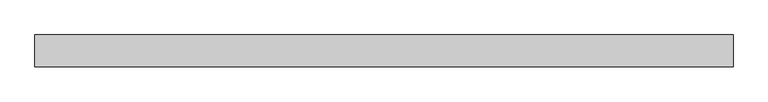
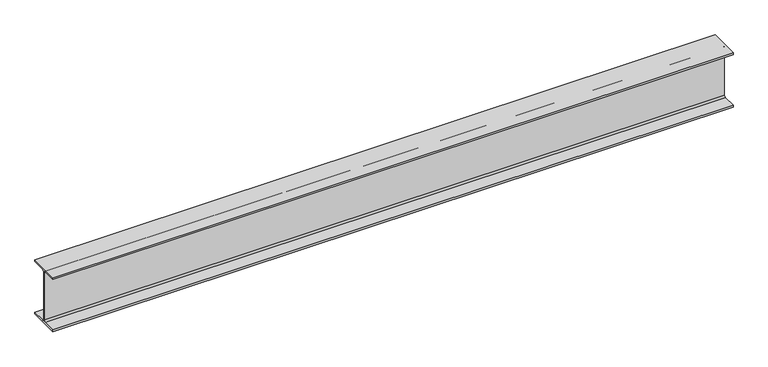
"""IFC4 building model written with IfcOpenShell, lengths in millimetres: beam geometry, Old_Steel Beam_H-KSD3502 : H_SB_ASB_H-200×200x8x12."""

from ifc_helpers import new_model, si_unit, point, frame, frame_2d, origin, place, context, project, spatial, polyline, circle_curve, trimmed, segment, composite_curve, outline, extrude, source, transform, mapped, element, save


def beam_a9061e91(model_context):
    return source(origin(), model_context, "Body", "SweptSolid", [
        extrude(outline(composite_curve([segment(polyline([(82.5, -141.5), (82.5, -151.7), (-82.5, -151.7), (-82.5, -141.5), (-11.9, -141.5)]), True, "CONTINUOUS"), segment(trimmed(circle_curve(frame_2d((-11.9, -132.6)), 8.9), [point((-11.9, -141.5))], [point((-3.0, -132.6))], True, "CARTESIAN"), True, "CONTINUOUS"), segment(polyline([(-3.0, -132.6), (-3.0, 132.6)]), True, "CONTINUOUS"), segment(trimmed(circle_curve(frame_2d((-11.9, 132.6)), 8.9), [point((-3.0, 132.6))], [point((-11.9, 141.5))], True, "CARTESIAN"), True, "CONTINUOUS"), segment(polyline([(-11.9, 141.5), (-82.5, 141.5), (-82.5, 151.7), (82.5, 151.7), (82.5, 141.5), (11.9, 141.5)]), True, "CONTINUOUS"), segment(trimmed(circle_curve(frame_2d((11.9, 132.6)), 8.9), [point((11.9, 141.5))], [point((3.0, 132.6))], True, "CARTESIAN"), True, "CONTINUOUS"), segment(polyline([(3.0, 132.6), (3.0, -132.6)]), True, "CONTINUOUS"), segment(trimmed(circle_curve(frame_2d((11.9, -132.6)), 8.9), [point((3.0, -132.6))], [point((11.9, -141.5))], True, "CARTESIAN"), True, "CONTINUOUS"), segment(polyline([(11.9, -141.5), (82.5, -141.5)]), True, "CONTINUOUS")], self_intersect=False)), frame((-1890.900922, 0.0, 0.0), z_axis=(1.0, 0.0, 0.0), x_axis=(0.0, 1.0, 0.0)), (0.0, 0.0, 1.0), 3596.321771),
    ])


if __name__ == "__main__":
    model = new_model("IFC4")
    model_context = context("Model", 3, world=origin())
    ifc_project = project(units=[si_unit("LENGTHUNIT", "METRE", prefix="MILLI")], contexts=[model_context])
    site = spatial("IfcSite", under=ifc_project)
    building = spatial("IfcBuilding", under=site)
    placement = place(None, origin())
    beam_shape = beam_a9061e91(model_context)
    element("IfcBeam", 1, ObjectType="Old_Steel Beam_H-KSD3502 : H_SB_ASB_H-200×200x8x12", at=placement, inside=building, context=model_context, shape_type="MappedRepresentation", body=[
        mapped(beam_shape, transform((0.0, 0.0, 0.0), x_axis=(1.0, 0.0, 0.0), y_axis=(0.0, 1.0, 0.0), z_axis=(0.0, 0.0, 1.0))),
    ])
    save(model, "model.ifc")

# Revit data of these elements
# Type "Old_Steel Beam_H-KSD3502 : H_SB_ASB_H-200×200x8x12"
#   Width = 20.0 cm
#   Web Thickness = 0.8 cm
#   Web Fillet = 1.3 cm
#   Warping Constant = 141376.0 cm⁶
#   Torsional Moment of Inertia = 26.2485 cm⁴
#   Torsional Modulus = 1.0 cm³
#   Section Area = 63.53 cm²
#   Plastic Modulus weak axis = 244.0 cm³
#   Plastic Modulus strong axis = 525.0 cm³
#   Perimeter = 1.16 m²/m
#   Nominal Weight = 49.90 kgf/m
#   Moment of Inertia weak axis = 1600.00 cm⁴
#   Moment of Inertia strong axis = 4720.00 cm⁴
#   Height = 20.0 cm
#   Flange Thickness = 1.2 cm
#   Elastic Modulus weak axis = 160.0 cm³
#   Elastic Modulus strong axis = 472.0 cm³
#   Centroid Vertical = 10.0 cm
#   Centroid Horizontal = 10.0 cm
#   Length [instance default] = 1.5240 m
#   Structural Material [instance default] = Steel, 45-345
#   Assembly Code = ""
# Element 1 (IfcBeam, "Old_Steel Beam_H-KSD3502 : H_SB_ASB_H-200×200x8x12")
#   Structural Material = none
# Materials
#   "Steel, 45-345": class "Metal", colour RGB 189 187 185, transparency 0, Description = "Steel 345 MPa", Cost = 0
